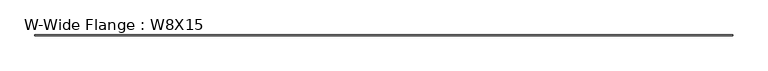
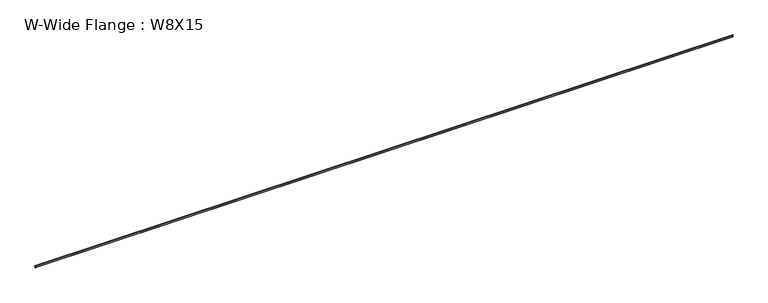
"""IFC4 building model written with IfcOpenShell, lengths in millimetres: beam geometry, W-Wide Flange : W8X15."""

from ifc_helpers import new_model, si_unit, point, frame, frame_2d, origin, place, context, project, spatial, polyline, circle_curve, trimmed, segment, composite_curve, outline, extrude, source, transform, mapped, element, save


def w_wide_flange_w8x15_6c148e4e(model_context):
    return source(origin(), model_context, "Body", "SweptSolid", [
        extrude(outline(composite_curve([segment(polyline([(50.927, -94.996), (50.927, -102.997), (-50.927, -102.997), (-50.927, -94.996), (-15.748, -94.996)]), True, "CONTINUOUS"), segment(trimmed(circle_curve(frame_2d((-15.748, -82.3595)), 12.6365), [point((-15.748, -94.996))], [point((-3.1115, -82.3595))], True, "CARTESIAN"), True, "CONTINUOUS"), segment(polyline([(-3.1115, -82.3595), (-3.1115, 82.3595)]), True, "CONTINUOUS"), segment(trimmed(circle_curve(frame_2d((-15.748, 82.3595)), 12.6365), [point((-3.1115, 82.3595))], [point((-15.748, 94.996))], True, "CARTESIAN"), True, "CONTINUOUS"), segment(polyline([(-15.748, 94.996), (-50.927, 94.996), (-50.927, 102.997), (50.927, 102.997), (50.927, 94.996), (15.748, 94.996)]), True, "CONTINUOUS"), segment(trimmed(circle_curve(frame_2d((15.748, 82.3595)), 12.6365), [point((15.748, 94.996))], [point((3.1115, 82.3595))], True, "CARTESIAN"), True, "CONTINUOUS"), segment(polyline([(3.1115, 82.3595), (3.1115, -82.3595)]), True, "CONTINUOUS"), segment(trimmed(circle_curve(frame_2d((15.748, -82.3595)), 12.6365), [point((3.1115, -82.3595))], [point((15.748, -94.996))], True, "CARTESIAN"), True, "CONTINUOUS"), segment(polyline([(15.748, -94.996), (50.927, -94.996)]), True, "CONTINUOUS")], self_intersect=False)), frame((-44289.8957353, 0.0, 0.0), z_axis=(1.0, 0.0, 0.0), x_axis=(0.0, 1.0, 0.0)), (0.0, 0.0, 1.0), 88692.2707353),
    ])


if __name__ == "__main__":
    model = new_model("IFC4")
    model_context = context("Model", 3, world=origin())
    ifc_project = project(units=[si_unit("LENGTHUNIT", "METRE", prefix="MILLI")], contexts=[model_context])
    site = spatial("IfcSite", under=ifc_project)
    building = spatial("IfcBuilding", under=site)
    placement = place(None, origin())
    w_wide_flange_w8x15_shape = w_wide_flange_w8x15_6c148e4e(model_context)
    element("IfcBeam", 1, ObjectType="W-Wide Flange : W8X15", at=placement, inside=building, context=model_context, shape_type="MappedRepresentation", body=[
        mapped(w_wide_flange_w8x15_shape, transform((0.0, 0.0, 0.0), x_axis=(1.0, 0.0, 0.0), y_axis=(0.0, 1.0, 0.0), z_axis=(0.0, 0.0, 1.0))),
    ])
    save(model, "model.ifc")

# Revit data of these elements
# Type "W-Wide Flange : W8X15"
#   Assembly Code = "B10"
#   W = 15
#   Length [instance default] = 5' - 0"
#   bf = 0' - 4.01"
#   d = 0' - 8.11"
#   k = 0' - 0 13/16"
#   k2 = 0' - 0.4975"
#   tf = 0' - 0.315"
#   tw = 0' - 0.245"
#   A = 0.0308333 SF
#   Structural Material [instance default] = Steel ASTM A992
# Element 1 (IfcBeam, "W-Wide Flange : W8X15")
#   Materials on its faces: "Steel ASTM A992"
# Materials
#   "Steel ASTM A992": class "Metal", colour RGB 199 199 199, transparency 0, Description = "Structural steel 50ksi", Cost = 0
